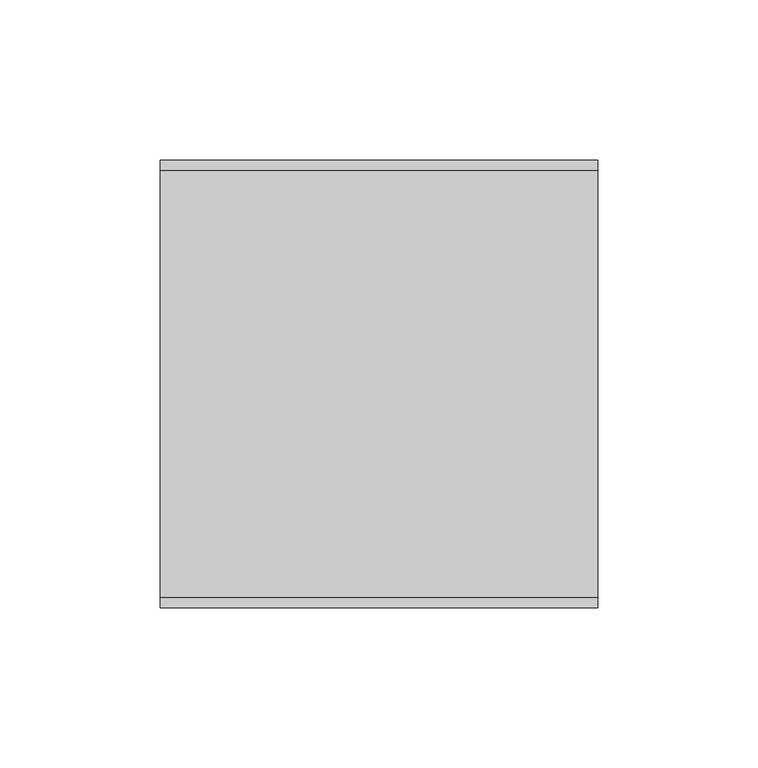
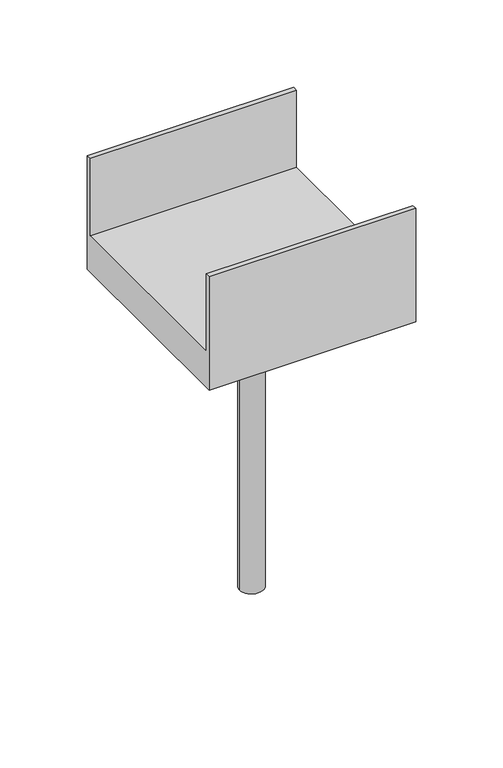
"""IFC4 building model written with IfcOpenShell, lengths in millimetres: fastener geometry."""

from ifc_helpers import new_model, si_unit, point, frame, origin, origin_with_axes, origin_2d, place, context, project, spatial, polyline, circle_curve, trimmed, segment, composite_curve, outline, extrude, source, transform, mapped, element, save


def fastener_ec502d19(model_context):
    return source(origin(), model_context, "Body", "SweptSolid", [
        extrude(outline(composite_curve([segment(trimmed(circle_curve(origin_2d(), 7.9375), [point((-7.9375, 0.0))], [point((7.9375, 0.0))], False, "CARTESIAN"), True, "CONTINUOUS"), segment(trimmed(circle_curve(origin_2d(), 7.9375), [point((7.9375, 0.0))], [point((-7.9375, 0.0))], False, "CARTESIAN"), True, "CONTINUOUS")], self_intersect=False)), frame((0.0, 0.0, -203.2), z_axis=(0.0, 0.0, 1.0), x_axis=(1.0, 0.0, 0.0)), (0.0, 0.0, 1.0), 203.2),
        extrude(outline(polyline([(-11.90625, -6.8740766), (-11.90625, 6.8740766), (0.0, 13.7481533), (11.90625, 6.8740766), (11.90625, -6.8740766), (0.0, -13.7481533), (-11.90625, -6.8740766)])), origin_with_axes(), (0.0, 0.0, 1.0), 11.2117187),
        extrude(outline(polyline([(69.85, 79.375), (69.85, 0.0), (-69.85, 0.0), (-69.85, 79.375), (-66.675, 79.375), (-66.675, 25.4), (66.675, 25.4), (66.675, 79.375), (69.85, 79.375)])), frame((-68.2625, 0.0, 0.0), z_axis=(1.0, 0.0, 0.0), x_axis=(0.0, 1.0, 0.0)), (0.0, 0.0, 1.0), 136.525),
    ])


if __name__ == "__main__":
    model = new_model("IFC4")
    model_context = context("Model", 3, world=origin())
    ifc_project = project(units=[si_unit("LENGTHUNIT", "METRE", prefix="MILLI")], contexts=[model_context])
    site = spatial("IfcSite", under=ifc_project)
    building = spatial("IfcBuilding", under=site)
    placement = place(None, origin())
    fastener_shape = fastener_ec502d19(model_context)
    element("IfcFastener", 1, ObjectType="SIMPSON - ABA- POST BASE : SIMPSON - ABA66Z W/ 5/8\"X8\" ANCHOR BOLT W/ NON-SHRINK GROUT AT BASE", at=placement, inside=building, context=model_context, shape_type="MappedRepresentation", body=[
        mapped(fastener_shape, transform((0.0, 0.0, 0.0), x_axis=(1.0, 0.0, 0.0), y_axis=(0.0, 1.0, 0.0), z_axis=(0.0, 0.0, 1.0))),
    ])
    save(model, "model.ifc")

# Revit data of these elements
# Type "SIMPSON - ABA- POST BASE : SIMPSON - ABA66Z W/ 5/8\"X8\" ANCHOR BOLT W/ NON-SHRINK GROUT AT BASE"
#   L = 0' - 3"
#   Hole Radius = 0' - 0 3/8"
#   D4 = 0' - 5"
#   D2 = 0' - 5"
#   D1 = 0' - 1 1/2"
#   D3 = 0' - 2 3/4"
#   Ga. = 0' - 0 61/256"
#   W1 & W2 = 0' - 4 1/4"
#   Default Elevation = 4' - 0"
#   Bolt Visibility - 3B = no
#   Bolt Visibility - 3A = no
#   Bolt Visibility - 2B = no
#   Bolt Visibility - 2A = no
#   Bolt Visibility - 1B = no
#   Bolt Visibility - 1A = yes
#   Bolt Visibility = yes
#   Material = ABA66Z W/ 5/8"X8" ANCHOR BOLT W/ NON-SHRINK GROUT AT BASE
#   Bolt Size = element 1605874
#   URL = ""
# Element 1 (IfcFastener, "SIMPSON - ABA- POST BASE : SIMPSON - ABA66Z W/ 5/8\"X8\" ANCHOR BOLT W/ NON-SHRINK GROUT AT BASE")
#   Materials on its faces: "1\" GALV. LAG BOLT (LENGTH = 1/2\" SHY OF GLULAM DEPTH) -  (GALV. THRU BOLT IF PLATE ON OPP. SIDE OF STRUCT MEMBER)", "ABA66Z W/ 5/8\"X8\" ANCHOR BOLT W/ NON-SHRINK GROUT AT BASE"
# Materials
#   "ABA66Z W/ 5/8\"X8\" ANCHOR BOLT W/ NON-SHRINK GROUT AT BASE": class "Generic", colour RGB 232 232 232, transparency 0, Cost = 0
#   "1\" GALV. LAG BOLT (LENGTH = 1/2\" SHY OF GLULAM DEPTH) -  (GALV. THRU BOLT IF PLATE ON OPP. SIDE OF STRUCT MEMBER)": class "Generic", colour RGB 120 120 120, transparency 0, Cost = 0
